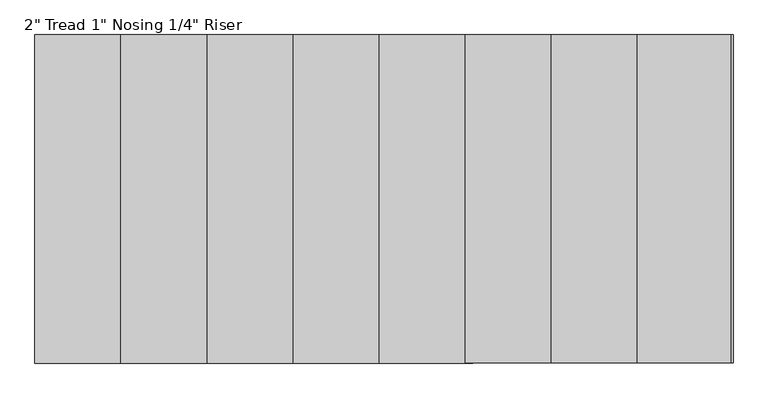
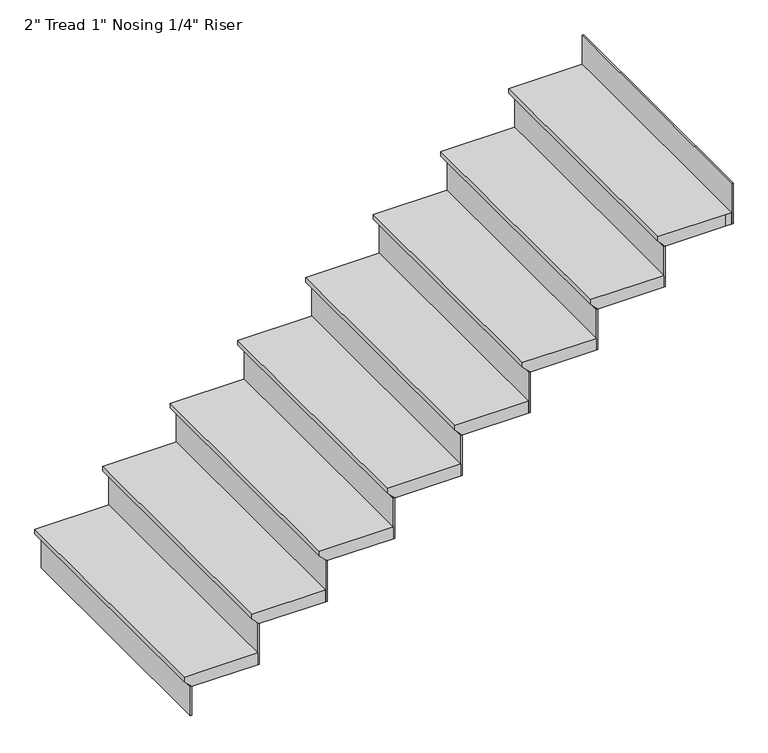
"""IFC4 building model written with IfcOpenShell, lengths in millimetres: stair flight geometry."""

from ifc_helpers import new_model, si_unit, origin, place, context, project, spatial, faceted_brep, source, transform, mapped, element, save


def stair_flight_d277631b(model_context):
    return source(origin(), model_context, "Body", "Brep", [
        faceted_brep([(663721.188677, -551651.2413841, 158.0635135), (663721.188677, -551651.2413841, 177.1135135), (663721.188677, -550584.4413841, 177.1135135), (663721.188677, -550584.4413841, 158.0635135), (663746.588677, -551651.2413841, 132.6635135), (663746.588677, -550584.4413841, 132.6635135), (664025.988677, -551651.2413841, 177.1135135), (664025.988677, -550584.4413841, 177.1135135), (663746.588677, -550584.4413841, 126.3135135), (664025.988677, -550584.4413841, 126.3135135), (664025.988677, -551651.2413841, 126.3135135), (663746.588677, -551651.2413841, 126.3135135)], [[[0, 1, 2, 3]], [[4, 0, 3, 5]], [[2, 1, 6, 7]], [[8, 9, 10, 11]], [[2, 7, 9, 8, 5, 3]], [[8, 11, 4, 5]], [[6, 1, 0, 4, 11, 10]], [[7, 6, 10, 9]]]),
        faceted_brep([(663746.588677, -551651.2413841, 126.3135135), (663746.588677, -551651.2413841, 0.0), (663752.938677, -551651.2413841, 0.0), (663752.938677, -551651.2413841, 126.3135135), (663746.588677, -550584.4413841, 126.3135135), (663752.938677, -550584.4413841, 126.3135135), (663752.938677, -550584.4413841, 0.0), (663746.588677, -550584.4413841, 0.0)], [[[0, 1, 2, 3]], [[4, 5, 6, 7]], [[1, 0, 4, 7]], [[2, 1, 7, 6]], [[3, 2, 6, 5]], [[0, 3, 5, 4]]]),
        faceted_brep([(664025.988677, -551651.2413841, 303.427027), (664025.988677, -551651.2413841, 126.3135135), (664032.338677, -551651.2413841, 126.3135135), (664032.338677, -551651.2413841, 303.427027), (664025.988677, -550584.4413841, 303.427027), (664032.338677, -550584.4413841, 303.427027), (664032.338677, -550584.4413841, 126.3135135), (664025.988677, -550584.4413841, 126.3135135)], [[[0, 1, 2, 3]], [[4, 5, 6, 7]], [[1, 0, 4, 7]], [[2, 1, 7, 6]], [[3, 2, 6, 5]], [[0, 3, 5, 4]]]),
        faceted_brep([(664000.588677, -550584.4413841, 354.227027), (664000.588677, -551651.2413841, 354.227027), (664305.388677, -551651.2413841, 354.227027), (664305.388677, -550584.4413841, 354.227027), (664025.988677, -550584.4413841, 303.427027), (664305.388677, -550584.4413841, 303.427027), (664305.388677, -551651.2413841, 303.427027), (664025.988677, -551651.2413841, 303.427027), (664025.988677, -550584.4413841, 309.777027), (664000.588677, -550584.4413841, 335.177027), (664025.988677, -551651.2413841, 309.777027), (664000.588677, -551651.2413841, 335.177027)], [[[0, 1, 2, 3]], [[4, 5, 6, 7]], [[0, 3, 5, 4, 8, 9]], [[4, 7, 10, 8]], [[2, 1, 11, 10, 7, 6]], [[3, 2, 6, 5]], [[11, 1, 0, 9]], [[10, 11, 9, 8]]]),
        faceted_brep([(664305.388677, -551651.2413841, 480.5405405), (664305.388677, -551651.2413841, 303.427027), (664311.738677, -551651.2413841, 303.427027), (664311.738677, -551651.2413841, 480.5405405), (664305.388677, -550584.4413841, 480.5405405), (664311.738677, -550584.4413841, 480.5405405), (664311.738677, -550584.4413841, 303.427027), (664305.388677, -550584.4413841, 303.427027)], [[[0, 1, 2, 3]], [[4, 5, 6, 7]], [[1, 0, 4, 7]], [[2, 1, 7, 6]], [[3, 2, 6, 5]], [[0, 3, 5, 4]]]),
        faceted_brep([(664279.988677, -550584.4413841, 531.3405405), (664279.988677, -551651.2413841, 531.3405405), (664584.788677, -551651.2413841, 531.3405405), (664584.788677, -550584.4413841, 531.3405405), (664305.388677, -550584.4413841, 480.5405405), (664584.788677, -550584.4413841, 480.5405405), (664584.788677, -551651.2413841, 480.5405405), (664305.388677, -551651.2413841, 480.5405405), (664305.388677, -550584.4413841, 486.8905405), (664279.988677, -550584.4413841, 512.2905405), (664305.388677, -551651.2413841, 486.8905405), (664279.988677, -551651.2413841, 512.2905405)], [[[0, 1, 2, 3]], [[4, 5, 6, 7]], [[0, 3, 5, 4, 8, 9]], [[4, 7, 10, 8]], [[2, 1, 11, 10, 7, 6]], [[3, 2, 6, 5]], [[11, 1, 0, 9]], [[10, 11, 9, 8]]]),
        faceted_brep([(664584.788677, -551651.2413841, 657.6540541), (664584.788677, -551651.2413841, 480.5405405), (664591.138677, -551651.2413841, 480.5405405), (664591.138677, -551651.2413841, 657.6540541), (664584.788677, -550584.4413841, 657.6540541), (664591.138677, -550584.4413841, 657.6540541), (664591.138677, -550584.4413841, 480.5405405), (664584.788677, -550584.4413841, 480.5405405)], [[[0, 1, 2, 3]], [[4, 5, 6, 7]], [[1, 0, 4, 7]], [[2, 1, 7, 6]], [[3, 2, 6, 5]], [[0, 3, 5, 4]]]),
        faceted_brep([(664559.388677, -550584.4413841, 708.4540541), (664559.388677, -551651.2413841, 708.4540541), (664864.188677, -551651.2413841, 708.4540541), (664864.188677, -550584.4413841, 708.4540541), (664584.788677, -550584.4413841, 657.6540541), (664864.188677, -550584.4413841, 657.6540541), (664864.188677, -551651.2413841, 657.6540541), (664584.788677, -551651.2413841, 657.6540541), (664584.788677, -550584.4413841, 664.0040541), (664559.388677, -550584.4413841, 689.4040541), (664584.788677, -551651.2413841, 664.0040541), (664559.388677, -551651.2413841, 689.4040541)], [[[0, 1, 2, 3]], [[4, 5, 6, 7]], [[0, 3, 5, 4, 8, 9]], [[4, 7, 10, 8]], [[2, 1, 11, 10, 7, 6]], [[3, 2, 6, 5]], [[11, 1, 0, 9]], [[10, 11, 9, 8]]]),
        faceted_brep([(664864.188677, -551651.2413841, 834.7675676), (664864.188677, -551651.2413841, 657.6540541), (664870.538677, -551651.2413841, 657.6540541), (664870.538677, -551651.2413841, 834.7675676), (664864.188677, -550584.4413841, 834.7675676), (664870.538677, -550584.4413841, 834.7675676), (664870.538677, -550584.4413841, 657.6540541), (664864.188677, -550584.4413841, 657.6540541)], [[[0, 1, 2, 3]], [[4, 5, 6, 7]], [[1, 0, 4, 7]], [[2, 1, 7, 6]], [[3, 2, 6, 5]], [[0, 3, 5, 4]]]),
        faceted_brep([(664838.788677, -550584.4413841, 885.5675676), (664838.788677, -551651.2413841, 885.5675676), (665143.588677, -551651.2413841, 885.5675676), (665143.588677, -550584.4413841, 885.5675676), (664864.188677, -550584.4413841, 834.7675676), (665143.588677, -550584.4413841, 834.7675676), (665143.588677, -551651.2413841, 834.7675676), (664864.188677, -551651.2413841, 834.7675676), (664864.188677, -550584.4413841, 841.1175676), (664838.788677, -550584.4413841, 866.5175676), (664864.188677, -551651.2413841, 841.1175676), (664838.788677, -551651.2413841, 866.5175676)], [[[0, 1, 2, 3]], [[4, 5, 6, 7]], [[0, 3, 5, 4, 8, 9]], [[4, 7, 10, 8]], [[2, 1, 11, 10, 7, 6]], [[3, 2, 6, 5]], [[11, 1, 0, 9]], [[10, 11, 9, 8]]]),
        faceted_brep([(665143.588677, -551651.2413841, 1011.8810811), (665143.588677, -551651.2413841, 834.7675676), (665149.938677, -551651.2413841, 834.7675676), (665149.938677, -551651.2413841, 1011.8810811), (665143.588677, -550584.4413841, 1011.8810811), (665149.938677, -550584.4413841, 1011.8810811), (665149.938677, -550584.4413841, 834.7675676), (665143.588677, -550584.4413841, 834.7675676)], [[[0, 1, 2, 3]], [[4, 5, 6, 7]], [[1, 0, 4, 7]], [[2, 1, 7, 6]], [[3, 2, 6, 5]], [[0, 3, 5, 4]]]),
        faceted_brep([(665118.188677, -550584.4413841, 1062.6810811), (665118.188677, -551651.2413841, 1062.6810811), (665422.988677, -551651.2413841, 1062.6810811), (665422.988677, -550584.4413841, 1062.6810811), (665143.588677, -550584.4413841, 1011.8810811), (665422.988677, -550584.4413841, 1011.8810811), (665422.988677, -551651.2413841, 1011.8810811), (665143.588677, -551651.2413841, 1011.8810811), (665143.588677, -550584.4413841, 1018.2310811), (665118.188677, -550584.4413841, 1043.6310811), (665143.588677, -551651.2413841, 1018.2310811), (665118.188677, -551651.2413841, 1043.6310811)], [[[0, 1, 2, 3]], [[4, 5, 6, 7]], [[0, 3, 5, 4, 8, 9]], [[4, 7, 10, 8]], [[2, 1, 11, 10, 7, 6]], [[3, 2, 6, 5]], [[11, 1, 0, 9]], [[10, 11, 9, 8]]]),
        faceted_brep([(665422.988677, -551651.2413841, 1188.9945946), (665422.988677, -551651.2413841, 1011.8810811), (665429.338677, -551651.2413841, 1011.8810811), (665429.338677, -551651.2413841, 1188.9945946), (665422.988677, -550584.4413841, 1188.9945946), (665429.338677, -550584.4413841, 1188.9945946), (665429.338677, -550584.4413841, 1011.8810811), (665422.988677, -550584.4413841, 1011.8810811)], [[[0, 1, 2, 3]], [[4, 5, 6, 7]], [[1, 0, 4, 7]], [[2, 1, 7, 6]], [[3, 2, 6, 5]], [[0, 3, 5, 4]]]),
        faceted_brep([(665397.588677, -550584.4413841, 1239.7945946), (665397.588677, -551651.2413841, 1239.7945946), (665702.388677, -551651.2413841, 1239.7945946), (665702.388677, -550584.4413841, 1239.7945946), (665422.988677, -550584.4413841, 1188.9945946), (665702.388677, -550584.4413841, 1188.9945946), (665702.388677, -551651.2413841, 1188.9945946), (665422.988677, -551651.2413841, 1188.9945946), (665422.988677, -550584.4413841, 1195.3445946), (665397.588677, -550584.4413841, 1220.7445946), (665422.988677, -551651.2413841, 1195.3445946), (665397.588677, -551651.2413841, 1220.7445946)], [[[0, 1, 2, 3]], [[4, 5, 6, 7]], [[0, 3, 5, 4, 8, 9]], [[4, 7, 10, 8]], [[2, 1, 11, 10, 7, 6]], [[3, 2, 6, 5]], [[11, 1, 0, 9]], [[10, 11, 9, 8]]]),
        faceted_brep([(665981.788677, -551651.2413841, 1543.2216216), (665981.788677, -551651.2413841, 1366.1081081), (665988.138677, -551651.2413841, 1366.1081081), (665988.138677, -551651.2413841, 1543.2216216), (665981.788677, -550584.4413841, 1543.2216216), (665988.138677, -550584.4413841, 1543.2216216), (665988.138677, -550584.4413841, 1366.1081081), (665981.788677, -550584.4413841, 1366.1081081)], [[[0, 1, 2, 3]], [[4, 5, 6, 7]], [[1, 0, 4, 7]], [[2, 1, 7, 6]], [[3, 2, 6, 5]], [[0, 3, 5, 4]]]),
        faceted_brep([(665702.388677, -551651.2413841, 1366.1081081), (665702.388677, -551651.2413841, 1188.9945946), (665708.738677, -551651.2413841, 1188.9945946), (665708.738677, -551651.2413841, 1366.1081081), (665702.388677, -550584.4413841, 1366.1081081), (665708.738677, -550584.4413841, 1366.1081081), (665708.738677, -550584.4413841, 1188.9945946), (665702.388677, -550584.4413841, 1188.9945946)], [[[0, 1, 2, 3]], [[4, 5, 6, 7]], [[1, 0, 4, 7]], [[2, 1, 7, 6]], [[3, 2, 6, 5]], [[0, 3, 5, 4]]]),
        faceted_brep([(665676.988677, -550584.4413841, 1416.9081081), (665676.988677, -551651.2413841, 1416.9081081), (665956.388677, -551651.2413841, 1416.9081081), (665981.788677, -551651.2413841, 1416.9081081), (665981.788677, -550584.4413841, 1416.9081081), (665702.388677, -550584.4413841, 1366.1081081), (665981.788677, -550584.4413841, 1366.1081081), (665981.788677, -551651.2413841, 1366.1081081), (665956.388677, -551651.2413841, 1366.1081081), (665702.388677, -551651.2413841, 1366.1081081), (665702.388677, -550584.4413841, 1372.4581081), (665676.988677, -550584.4413841, 1397.8581081), (665702.388677, -551651.2413841, 1372.4581081), (665676.988677, -551651.2413841, 1397.8581081)], [[[0, 1, 2, 3, 4]], [[5, 6, 7, 8, 9]], [[0, 4, 6, 5, 10, 11]], [[5, 9, 12, 10]], [[2, 1, 13, 12, 9, 8]], [[3, 2, 8, 7]], [[4, 3, 7, 6]], [[13, 1, 0, 11]], [[12, 13, 11, 10]]]),
    ])


if __name__ == "__main__":
    model = new_model("IFC4")
    model_context = context("Model", 3, world=origin())
    ifc_project = project(units=[si_unit("LENGTHUNIT", "METRE", prefix="MILLI")], contexts=[model_context])
    site = spatial("IfcSite", under=ifc_project)
    building = spatial("IfcBuilding", under=site)
    placement = place(None, origin())
    stair_flight_shape = stair_flight_d277631b(model_context)
    element("IfcStairFlight", 1, ObjectType="2\" Tread 1\" Nosing 1/4\" Riser", at=placement, inside=building, context=model_context, shape_type="MappedRepresentation", body=[
        mapped(stair_flight_shape, transform((0.0, 0.0, 0.0), x_axis=(1.0, 0.0, 0.0), y_axis=(0.0, 1.0, 0.0), z_axis=(0.0, 0.0, 1.0))),
    ])
    save(model, "model.ifc")
